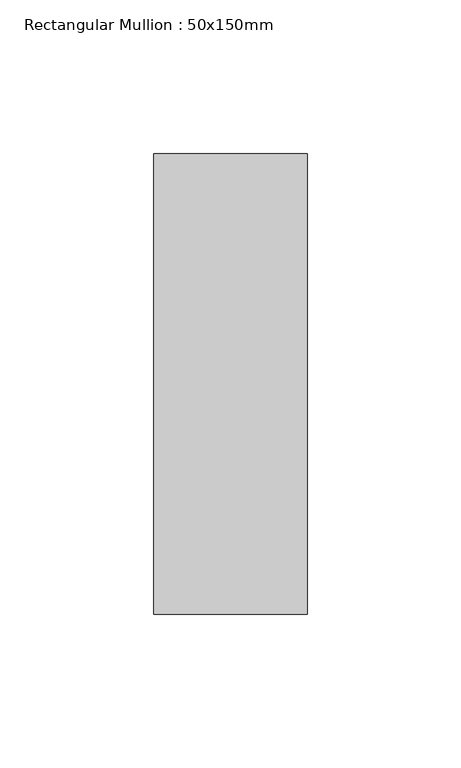
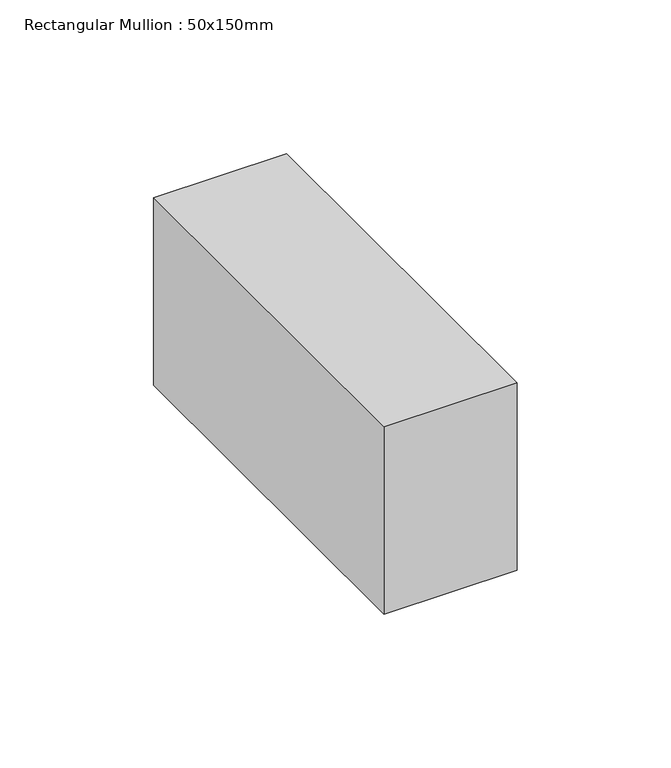
"""IFC4 building model written with IfcOpenShell, lengths in millimetres: member geometry, Rectangular Mullion : 50x150mm."""

from ifc_helpers import new_model, si_unit, frame, origin, place, context, project, spatial, polyline, outline, extrude, source, transform, mapped, element, save


def rectangular_mullion_50x150mm_0166ad73(model_context):
    return source(origin(), model_context, "Body", "SweptSolid", [
        extrude(outline(polyline([(25.0, 75.0), (25.0, -75.0), (-25.0, -75.0), (-25.0, 75.0), (25.0, 75.0)])), frame((0.0, 0.0, -74.4185145), z_axis=(0.0, 0.0, 1.0), x_axis=(1.0, 0.0, 0.0)), (0.0, 0.0, 1.0), 74.4185145),
    ])


if __name__ == "__main__":
    model = new_model("IFC4")
    model_context = context("Model", 3, world=origin())
    ifc_project = project(units=[si_unit("LENGTHUNIT", "METRE", prefix="MILLI")], contexts=[model_context])
    site = spatial("IfcSite", under=ifc_project)
    building = spatial("IfcBuilding", under=site)
    placement = place(None, origin())
    rectangular_mullion_50x150mm_shape = rectangular_mullion_50x150mm_0166ad73(model_context)
    element("IfcMember", 1, ObjectType="Rectangular Mullion : 50x150mm", at=placement, inside=building, context=model_context, shape_type="MappedRepresentation", body=[
        mapped(rectangular_mullion_50x150mm_shape, transform((0.0, 0.0, 0.0), x_axis=(1.0, 0.0, 0.0), y_axis=(0.0, 1.0, 0.0), z_axis=(0.0, 0.0, 1.0))),
    ])
    save(model, "model.ifc")

# Revit data of these elements
# Type "Rectangular Mullion : 50x150mm"
#   Keynote = "H11"
#   built-in parameter 1007304 = 0.492126 (stored number, unit not read)
#   built-in parameter 1007301 = 0.082021 (stored number, unit not read)
#   built-in parameter 1007300 = 0.082021 (stored number, unit not read)
# Element 1 (IfcMember, "Rectangular Mullion : 50x150mm")
#   Materials on its faces: "Aluminium"
# Materials
#   "Aluminium": class "Metal", colour RGB 247 247 247, transparency 0, Description = "Aluminium 6061", Cost = 0
